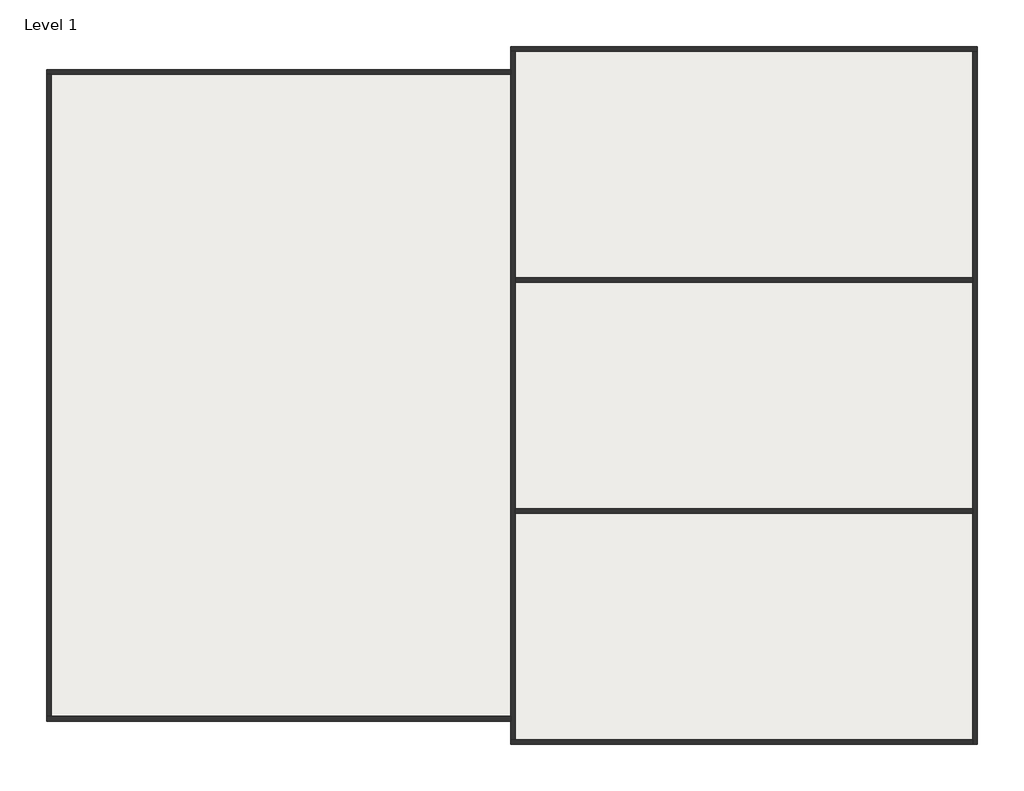
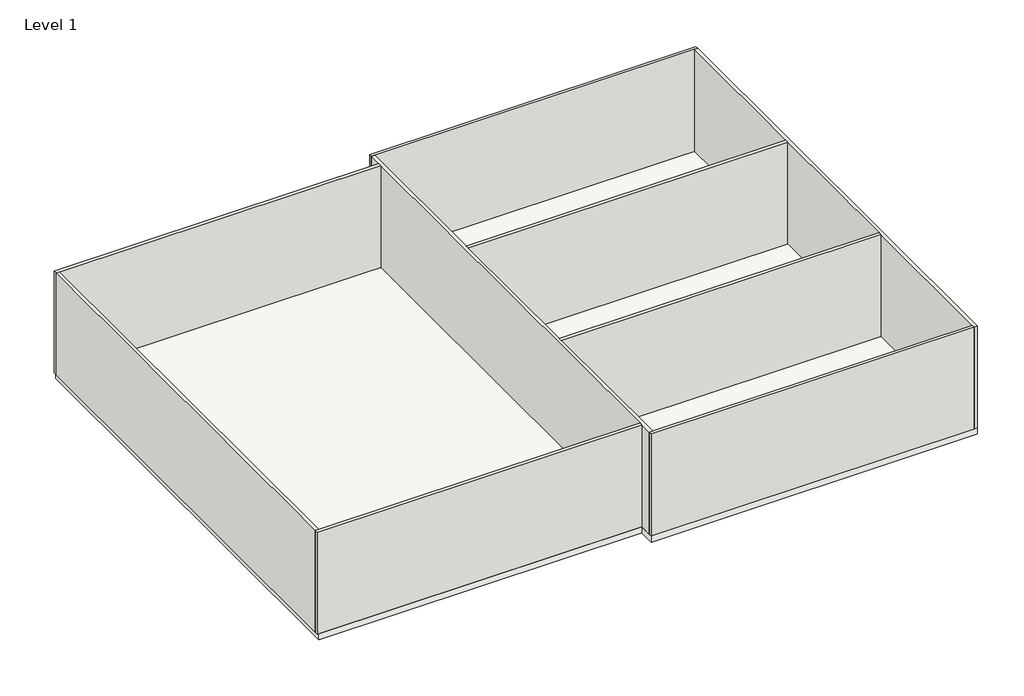
# One storey: 9 walls, 1 slab.
"""IFC4 building model written with IfcOpenShell, lengths in millimetres."""

from ifc_helpers import new_model, si_unit, frame, origin, origin_with_axes, place, context, project, spatial, polyline, outline, extrude, faceted_brep, element, save

model = new_model("IFC4")

# Units and contexts
model_context = context("Model", 3, world=origin())
ifc_project = project(units=[si_unit("LENGTHUNIT", "METRE", prefix="MILLI")], contexts=[model_context])

# Site, building, storey
site = spatial("IfcSite", under=ifc_project)
building = spatial("IfcBuilding", under=site)
storey = spatial("IfcBuildingStorey", under=building, Name="Level 1", Elevation=0.0)

# Slab
placement = place(None, origin())
element("IfcSlab", 1, ObjectType="Generic Floor - 400mm", at=placement, inside=storey, context=model_context, shape_type="SweptSolid", body=[
    extrude(outline(polyline([(15961.6453008, 15932.1645221), (15961.6453008, 16932.1645221), (36161.6453008, 16932.1645221), (36161.6453008, -13267.8354779), (15961.6453008, -13267.8354779), (15961.6453008, -12267.8354779), (-4038.3546992, -12267.8354779), (-4038.3546992, 15932.1645221), (15961.6453008, 15932.1645221)])), frame((0.0, 0.0, -400.0), z_axis=(0.0, 0.0, 1.0), x_axis=(1.0, 0.0, 0.0)), (0.0, 0.0, 1.0), 400.0),
])

# Walls
element("IfcWall", 2, ObjectType="Generic - 200mm", at=placement, inside=storey, context=model_context, shape_type="Brep", body=[
    faceted_brep([(16161.6453008, -13067.8354779, 0.0), (16161.6453008, -3267.8354779, 0.0), (16161.6453008, -3067.8354779, 0.0), (16161.6453008, 6732.1645221, 0.0), (16161.6453008, 6932.1645221, 0.0), (16161.6453008, 16732.1645221, 0.0), (16161.6453008, 16732.1645221, 6680.0), (16161.6453008, 6932.1645221, 6680.0), (16161.6453008, 6732.1645221, 6680.0), (16161.6453008, -3067.8354779, 6680.0), (16161.6453008, -3267.8354779, 6680.0), (16161.6453008, -13067.8354779, 6680.0), (15961.6453008, -13067.8354779, 0.0), (15961.6453008, -13067.8354779, 6680.0), (15961.6453008, -12267.8354779, 6680.0), (15961.6453008, -12067.8354779, 6680.0), (15961.6453008, 15732.1645221, 6680.0), (15961.6453008, 15932.1645221, 6680.0), (15961.6453008, 16732.1645221, 6680.0), (15961.6453008, 16732.1645221, 0.0), (15961.6453008, 15932.1645221, 0.0), (15961.6453008, 15732.1645221, 0.0), (15961.6453008, -12067.8354779, 0.0), (15961.6453008, -12267.8354779, 0.0)], [[[0, 1, 2, 3, 4, 5, 6, 7, 8, 9, 10, 11]], [[12, 13, 14, 15, 16, 17, 18, 19, 20, 21, 22, 23]], [[5, 4, 3, 2, 1, 0, 12, 23, 22, 21, 20, 19]], [[0, 11, 13, 12]], [[6, 5, 19, 18]], [[11, 10, 9, 8, 7, 6, 18, 17, 16, 15, 14, 13]]]),
])
element("IfcWall", 3, ObjectType="curtain wall - 200mm", at=placement, inside=storey, context=model_context, shape_type="Brep", body=[
    faceted_brep([(-4138.8546992, 15732.1645221, 0.0), (-3938.8546992, 15732.1645221, 0.0), (15961.6453008, 15732.1645221, 0.0), (15961.6453008, 15732.1645221, 6680.0), (-3938.8546992, 15732.1645221, 6680.0), (-4138.8546992, 15732.1645221, 6680.0), (-4138.8546992, 15932.1645221, 0.0), (-4138.8546992, 15932.1645221, 6680.0), (15961.6453008, 15932.1645221, 6680.0), (15961.6453008, 15932.1645221, 0.0)], [[[0, 1, 2, 3, 4, 5]], [[6, 7, 8, 9]], [[2, 1, 0, 6, 9]], [[0, 5, 7, 6]], [[3, 2, 9, 8]], [[5, 4, 3, 8, 7]]]),
])
element("IfcWall", 4, ObjectType="curtain wall - 200mm", at=placement, inside=storey, context=model_context, shape_type="Brep", body=[
    faceted_brep([(15961.6453008, 16732.1645221, 0.0), (16161.6453008, 16732.1645221, 0.0), (35961.6453008, 16732.1645221, 0.0), (36161.6453008, 16732.1645221, 0.0), (36161.6453008, 16732.1645221, 6680.0), (35961.6453008, 16732.1645221, 6680.0), (16161.6453008, 16732.1645221, 6680.0), (15961.6453008, 16732.1645221, 6680.0), (15961.6453008, 16932.1645221, 0.0), (15961.6453008, 16932.1645221, 6680.0), (36161.6453008, 16932.1645221, 6680.0), (36161.6453008, 16932.1645221, 0.0)], [[[0, 1, 2, 3, 4, 5, 6, 7]], [[8, 9, 10, 11]], [[3, 2, 1, 0, 8, 11]], [[4, 3, 11, 10]], [[0, 7, 9, 8]], [[7, 6, 5, 4, 10, 9]]]),
])
element("IfcWall", 5, ObjectType="curtain wall - 200mm", at=placement, inside=storey, context=model_context, shape_type="Brep", body=[
    faceted_brep([(35961.6453008, 16732.1645221, 0.0), (35961.6453008, 6932.1645221, 0.0), (35961.6453008, 6732.1645221, 0.0), (35961.6453008, -3067.8354779, 0.0), (35961.6453008, -3267.8354779, 0.0), (35961.6453008, -13067.8354779, 0.0), (35961.6453008, -13267.8354779, 0.0), (35961.6453008, -13267.8354779, 6680.0), (35961.6453008, -13067.8354779, 6680.0), (35961.6453008, -3267.8354779, 6680.0), (35961.6453008, -3067.8354779, 6680.0), (35961.6453008, 6732.1645221, 6680.0), (35961.6453008, 6932.1645221, 6680.0), (35961.6453008, 16732.1645221, 6680.0), (36161.6453008, 16732.1645221, 0.0), (36161.6453008, 16732.1645221, 6680.0), (36161.6453008, -13267.8354779, 6680.0), (36161.6453008, -13267.8354779, 0.0)], [[[0, 1, 2, 3, 4, 5, 6, 7, 8, 9, 10, 11, 12, 13]], [[14, 15, 16, 17]], [[6, 5, 4, 3, 2, 1, 0, 14, 17]], [[0, 13, 15, 14]], [[7, 6, 17, 16]], [[13, 12, 11, 10, 9, 8, 7, 16, 15]]]),
])
element("IfcWall", 6, ObjectType="curtain wall - 200mm", at=placement, inside=storey, context=model_context, shape_type="Brep", body=[
    faceted_brep([(35961.6453008, -13067.8354779, 0.0), (16161.6453008, -13067.8354779, 0.0), (15961.6453008, -13067.8354779, 0.0), (15961.6453008, -13067.8354779, 6680.0), (16161.6453008, -13067.8354779, 6680.0), (35961.6453008, -13067.8354779, 6680.0), (35961.6453008, -13267.8354779, 0.0), (35961.6453008, -13267.8354779, 6680.0), (15961.6453008, -13267.8354779, 6680.0), (15961.6453008, -13267.8354779, 0.0)], [[[0, 1, 2, 3, 4, 5]], [[6, 7, 8, 9]], [[2, 1, 0, 6, 9]], [[0, 5, 7, 6]], [[3, 2, 9, 8]], [[5, 4, 3, 8, 7]]]),
])
element("IfcWall", 7, ObjectType="curtain wall - 200mm", at=placement, inside=storey, context=model_context, shape_type="Brep", body=[
    faceted_brep([(15961.6453008, -12067.8354779, 0.0), (-3938.8546992, -12067.8354779, 0.0), (-4138.8546992, -12067.8354779, 0.0), (-4138.8546992, -12067.8354779, 6680.0), (-3938.8546992, -12067.8354779, 6680.0), (15961.6453008, -12067.8354779, 6680.0), (15961.6453008, -12267.8354779, 0.0), (15961.6453008, -12267.8354779, 6680.0), (-4138.8546992, -12267.8354779, 6680.0), (-4138.8546992, -12267.8354779, 0.0)], [[[0, 1, 2, 3, 4, 5]], [[6, 7, 8, 9]], [[2, 1, 0, 6, 9]], [[0, 5, 7, 6]], [[3, 2, 9, 8]], [[5, 4, 3, 8, 7]]]),
])
element("IfcWall", 8, ObjectType="curtain wall - 200mm", at=placement, inside=storey, context=model_context, shape_type="SweptSolid", body=[
    extrude(outline(polyline([(-3938.8546992, 15732.1645221), (-3938.8546992, -12067.8354779), (-4138.8546992, -12067.8354779), (-4138.8546992, 15732.1645221), (-3938.8546992, 15732.1645221)])), origin_with_axes(), (0.0, 0.0, 1.0), 6680.0),
])
element("IfcWall", 9, ObjectType="curtain wall - 200mm", at=placement, inside=storey, context=model_context, shape_type="SweptSolid", body=[
    extrude(outline(polyline([(35961.6453008, 6732.1645221), (16161.6453008, 6732.1645221), (16161.6453008, 6932.1645221), (35961.6453008, 6932.1645221), (35961.6453008, 6732.1645221)])), origin_with_axes(), (0.0, 0.0, 1.0), 6680.0),
])
element("IfcWall", 10, ObjectType="curtain wall - 200mm", at=placement, inside=storey, context=model_context, shape_type="SweptSolid", body=[
    extrude(outline(polyline([(35961.6453008, -3267.8354779), (16161.6453008, -3267.8354779), (16161.6453008, -3067.8354779), (35961.6453008, -3067.8354779), (35961.6453008, -3267.8354779)])), origin_with_axes(), (0.0, 0.0, 1.0), 6680.0),
])

save(model, "model.ifc")

# Revit data of these elements
# Project information
#   Project Issue Date = "Issue Date"
#   Project Status = "Project Status"
#   Client Name = "Owner"
#   Project Address = "Enter address here"
#   Project Name = "Project Name"
#   Project Number = "Project Number"
# Type "Generic Floor - 400mm"
#   Function = 0
#   Layers, outside or top first: 400 mm no material (function 1)
# Type "Generic - 200mm"
#   Layers, outside or top first: 200 mm no material (function 1)
# Type "curtain wall - 200mm"
#   Layers, outside or top first: 200 mm "Glass, Clear Glazing" (function 1)
# Element 1 (IfcSlab, "Generic Floor - 400mm")
#   Height Offset From Level = 0 mm
#   Phase Created = New Construction
#   Materials on its faces: "Default Floor"
# Element 2 (IfcWall, "Generic - 200mm")
#   Top Offset = 0 mm
#   Base Offset = 0 mm
#   wall height = 6680 mm
#   Phase Created = New Construction
#   Base Constraint = Level 1
#   Top Constraint = Level 2
#   Materials on its faces: "Default Wall"
# Elements 3, 5, 7, 8 (IfcWall, "curtain wall - 200mm")
#   Top Offset = 0 mm
#   Base Offset = 0 mm
#   wall height = 6680 mm
#   Phase Created = New Construction
#   Base Constraint = Level 1
#   Top Constraint = Level 2
#   Materials on its faces: "Glass, Clear Glazing"
# Elements 4, 6 (IfcWall, "curtain wall - 200mm")
#   Top Offset = 0 mm
#   Base Offset = 0 mm
#   wall height = 6680 mm
#   Phase Created = New Construction
#   Base Constraint = Level 1
#   Top Constraint = Level 2
#   Materials on its faces: "Glass, Clear Glazing", "Default Wall"
# Elements 9, 10 (IfcWall, "curtain wall - 200mm")
#   Top Offset = -320 mm
#   Base Offset = 0 mm
#   wall height = 6680 mm
#   Phase Created = New Construction
#   Base Constraint = Level 1
#   Top Constraint = Level 2
#   Materials on its faces: "Glass, Clear Glazing"
# Materials
#   "Glass, Clear Glazing": class "Glass", colour RGB 0 128 192, transparency 0.75, Description = "Clear glazing", Cost = 0
#   "Default Floor": class "Miscellaneous", colour RGB 127 127 127, transparency 0, Cost = 0
#   "Default Wall": class "Miscellaneous", colour RGB 128 128 128, transparency 0, Cost = 0
# Room at (6346.041, 1887.869) mm, phase "New Construction", upper level "Level 1", upper offset 7000 mm, lower offset 0 mm
#   Number = "6"
#   Name = "Room"
# Room at (26870.717, 12149.331) mm, phase "New Construction", upper level "Level 1", upper offset 7000 mm, lower offset 0 mm
#   Number = "8"
#   Name = "Room"
# Room at (26193.912, 1405.044) mm, phase "New Construction", upper level "Level 1", upper offset 7000 mm, lower offset 0 mm
#   Number = "9"
#   Name = "Room"
# Room at (25686.307, -8324.034) mm, phase "New Construction", upper level "Level 1", upper offset 7000 mm, lower offset 0 mm
#   Number = "10"
#   Name = "Room"
